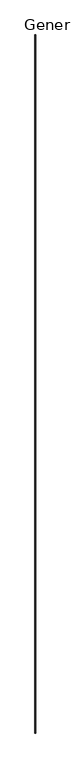
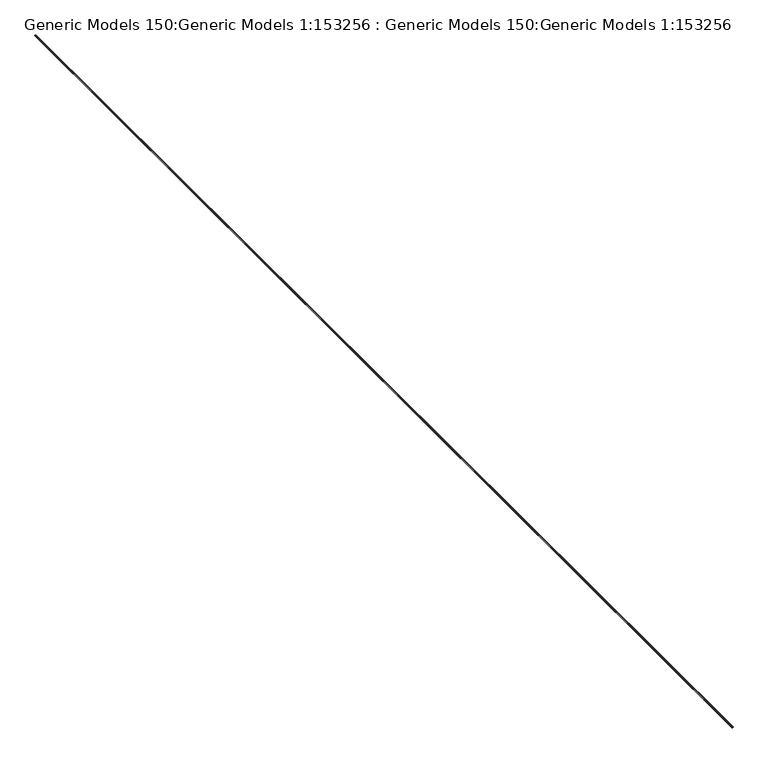
"""IFC4 building model written with IfcOpenShell, lengths in millimetres: proxy geometry, Generic Models 150:Generic Models 1:153256 : Generic Models 150:Generic Models 1:153256."""

from ifc_helpers import new_model, si_unit, point, frame, frame_2d, origin, place, context, project, spatial, polyline, circle_curve, trimmed, segment, composite_curve, outline, extrude, source, transform, mapped, element, save


def generic_models_150_generic_models_1_153256_generic_models_f4947532(model_context):
    return source(origin(), model_context, "Body", "SweptSolid", [
        extrude(outline(composite_curve([segment(trimmed(circle_curve(frame_2d((2890.6293287, -6658.751502)), 6.4650413), [point((2895.3918287, -6654.3793913))], [point((2885.8668287, -6654.3793913))], True, "CARTESIAN"), True, "CONTINUOUS"), segment(polyline([(2885.8668287, -6654.3793913), (2885.8668287, -6649.6168913)]), True, "CONTINUOUS"), segment(trimmed(circle_curve(frame_2d((2890.6293287, -6653.989002)), 6.4650413), [point((2885.8668287, -6649.6168913))], [point((2887.7728165, -6648.1892523))], False, "CARTESIAN"), True, "CONTINUOUS"), segment(polyline([(2887.7728165, -6648.1892523), (2887.0185822, -6647.1313395), (2886.4340937, -6645.8544386), (2886.0468287, -6644.4185785), (2885.8749931, -6642.8912608), (2885.9266651, -6641.3442868), (2886.1994154, -6639.8503818), (2886.6804218, -6638.4797761), (2887.3470715, -6637.2969037), (2888.1680244, -6636.3573731), (2889.1046864, -6635.7053527), (2890.1130239, -6635.371495), (2891.1456335, -6635.371495), (2892.153971, -6635.7053527), (2893.0906331, -6636.3573731), (2893.9115859, -6637.2969037), (2894.5782356, -6638.4797761), (2895.059242, -6639.8503818), (2895.3319923, -6641.3442868), (2895.3836643, -6642.8912608), (2895.2118287, -6644.4185785), (2894.8245637, -6645.8544386), (2894.2400753, -6647.1313395), (2893.4858409, -6648.1892523)]), True, "CONTINUOUS"), segment(trimmed(circle_curve(frame_2d((2890.6293287, -6653.989002)), 6.4650413), [point((2893.4858409, -6648.1892523))], [point((2895.3918287, -6649.6168913))], False, "CARTESIAN"), True, "CONTINUOUS"), segment(polyline([(2895.3918287, -6649.6168913), (2895.3918287, -6654.3793913)]), True, "CONTINUOUS")], self_intersect=False)), frame((0.0, -6877.9974793, 0.0), z_axis=(0.0, 1.0, 0.0), x_axis=(0.0, 0.0, 1.0)), (0.0, 0.0, 1.0), 19050.0),
    ])


if __name__ == "__main__":
    model = new_model("IFC4")
    model_context = context("Model", 3, world=origin())
    ifc_project = project(units=[si_unit("LENGTHUNIT", "METRE", prefix="MILLI")], contexts=[model_context])
    site = spatial("IfcSite", under=ifc_project)
    building = spatial("IfcBuilding", under=site)
    placement = place(None, origin())
    generic_models_150_generic_models_1_153256_generic_models_shape = generic_models_150_generic_models_1_153256_generic_models_f4947532(model_context)
    element("IfcBuildingElementProxy", 1, Name="Generic Models 150:Generic Models 1:153256 : Generic Models 150:Generic Models 1:153256", ObjectType="Generic Models 150:Generic Models 1:153256 : Generic Models 150:Generic Models 1:153256", at=placement, inside=building, context=model_context, shape_type="MappedRepresentation", body=[
        mapped(generic_models_150_generic_models_1_153256_generic_models_shape, transform((0.0, 0.0, 0.0), x_axis=(1.0, 0.0, 0.0), y_axis=(0.0, 1.0, 0.0), z_axis=(0.0, 0.0, 1.0))),
    ])
    save(model, "model.ifc")

# Revit data of these elements
# Type "Generic Models 150:Generic Models 1:153256 : Generic Models 150:Generic Models 1:153256"
#   NameOverride = "Generic Models 150:Generic Models 1:153256"
#   ObjectTypeOverride = "Generic Models 150:Generic Models 1"
#   Reference = "Generic Models 1"
#   Category = "Generic Models"
#   Tag = "153256"
# Element 1 (IfcBuildingElementProxy, "Generic Models 150:Generic Models 1:153256 : Generic Models 150:Generic Models 1:153256")
#   Materials on its faces: "_SEALANT AND BACKROD, IF NECESSARY 12051"
# Materials
#   "_SEALANT AND BACKROD, IF NECESSARY 12051": class "Unassigned", colour RGB 190 220 196, transparency 0
